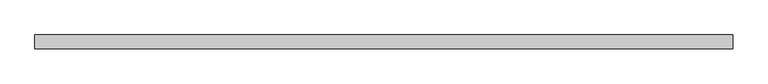
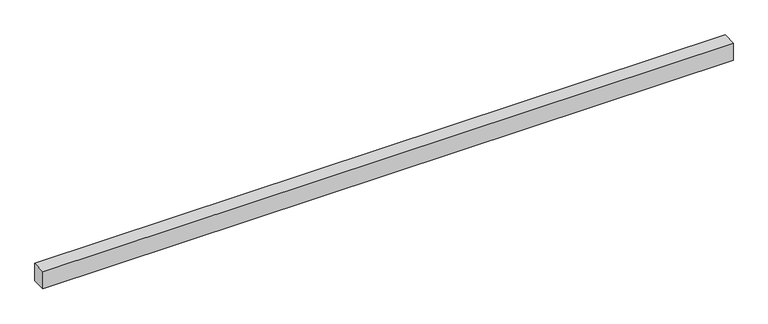
"""IFC4 building model written with IfcOpenShell, lengths in millimetres: proxy geometry, Generic Models 7:Generic Models 1:6:Generic Models 1:6 : Generic Models 7:Generic Models 1:337419:1 : Generic Models 7:Generic Models 1:6:Generic Models 1:6 : Generic Models 7:Generic Models 1:337419:312901."""

from ifc_helpers import new_model, si_unit, frame, origin, place, context, project, spatial, polyline, outline, extrude, source, transform, mapped, element, save


def generic_models_63b73bf6(model_context):
    return source(origin(), model_context, "Body", "SweptSolid", [
        extrude(outline(polyline([(-580032.0529717, -134.6760186), (-579142.0790656, -116.1348955), (-579142.0790656, -1293.8930223), (-580032.0529717, -1293.8930223), (-580032.0529717, -134.6760186)])), frame((557809.7867239, 0.0, 0.0), z_axis=(1.0, 0.0, 0.0), x_axis=(0.0, 1.0, 0.0)), (0.0, 0.0, 1.0), 44500.8),
    ])


if __name__ == "__main__":
    model = new_model("IFC4")
    model_context = context("Model", 3, world=origin())
    ifc_project = project(units=[si_unit("LENGTHUNIT", "METRE", prefix="MILLI")], contexts=[model_context])
    site = spatial("IfcSite", under=ifc_project)
    building = spatial("IfcBuilding", under=site)
    placement = place(None, origin())
    generic_models_shape = generic_models_63b73bf6(model_context)
    element("IfcBuildingElementProxy", 1, Name="Generic Models 7:Generic Models 1:6:Generic Models 1:6 : Generic Models 7:Generic Models 1:337419:1 : Generic Models 7:Generic Models 1:6:Generic Models 1:6 : Generic Models 7:Generic Models 1:337419:312901", ObjectType="Generic Models 7:Generic Models 1:6:Generic Models 1:6 : Generic Models 7:Generic Models 1:337419:1 : Generic Models 7:Generic Models 1:6:Generic Models 1:6 : Generic Models 7:Generic Models 1:337419:312901", at=placement, inside=building, context=model_context, shape_type="MappedRepresentation", body=[
        mapped(generic_models_shape, transform((0.0, 0.0, 0.0), x_axis=(1.0, 0.0, 0.0), y_axis=(0.0, 1.0, 0.0), z_axis=(0.0, 0.0, 1.0))),
    ])
    save(model, "model.ifc")

# Revit data of these elements
# Type "Generic Models 7:Generic Models 1:6:Generic Models 1:6 : Generic Models 7:Generic Models 1:337419:1 : Generic Models 7:Generic Models 1:6:Generic Models 1:6 : Generic Models 7:Generic Models 1:337419:312901"
#   NameOverride = "Generic Models 7:Generic Models 1:6:Generic Models 1:6 : Generic Models 7:Generic Models 1:337419:312901"
#   ObjectTypeOverride = "Generic Models 1:6 : Generic Models 7:Generic Models 1:337419"
#   Reference = "Generic Models 1"
#   Tag = "312901"
# Element 1 (IfcBuildingElementProxy, "Generic Models 7:Generic Models 1:6:Generic Models 1:6 : Generic Models 7:Generic Models 1:337419:1 : Generic Models 7:Generic Models 1:6:Generic Models 1:6 : Generic Models 7:Generic Models 1:337419:312901")
#   Materials on its faces: "GRADE"
# Materials
#   "GRADE": class "Generic", colour RGB 255 255 255, transparency 0, Cost = 0
